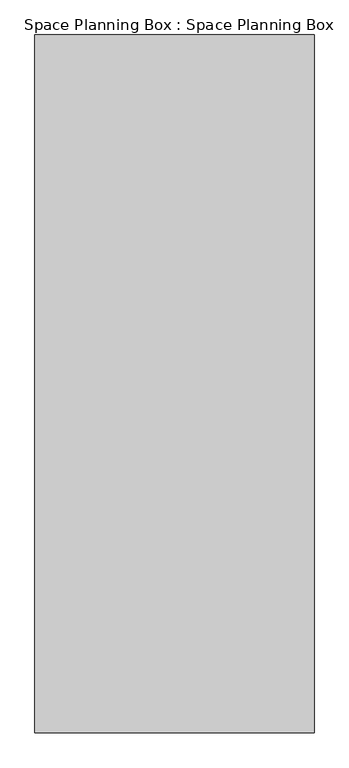
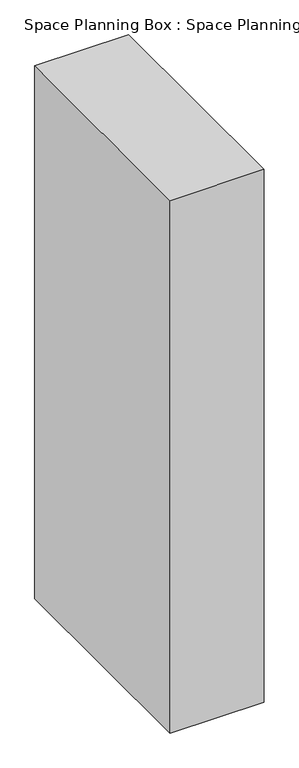
"""IFC4 building model written with IfcOpenShell, lengths in millimetres: proxy geometry, Space Planning Box : Space Planning Box."""

from ifc_helpers import new_model, si_unit, origin, origin_with_axes, place, context, project, spatial, polyline, outline, extrude, source, transform, mapped, element, save


def space_planning_box_space_planning_box_71e2440f(model_context):
    return source(origin(), model_context, "Body", "SweptSolid", [
        extrude(outline(polyline([(500.0, 1250.0), (500.0, -1250.0), (-500.0, -1250.0), (-500.0, 1250.0), (500.0, 1250.0)])), origin_with_axes(), (0.0, 0.0, 1.0), 6000.0),
    ])


if __name__ == "__main__":
    model = new_model("IFC4")
    model_context = context("Model", 3, world=origin())
    ifc_project = project(units=[si_unit("LENGTHUNIT", "METRE", prefix="MILLI")], contexts=[model_context])
    site = spatial("IfcSite", under=ifc_project)
    building = spatial("IfcBuilding", under=site)
    placement = place(None, origin())
    space_planning_box_space_planning_box_shape = space_planning_box_space_planning_box_71e2440f(model_context)
    element("IfcBuildingElementProxy", 1, Name="Space Planning Box : Space Planning Box", ObjectType="Space Planning Box : Space Planning Box", at=placement, inside=building, context=model_context, shape_type="MappedRepresentation", body=[
        mapped(space_planning_box_space_planning_box_shape, transform((0.0, 0.0, 0.0), x_axis=(1.0, 0.0, 0.0), y_axis=(0.0, 1.0, 0.0), z_axis=(0.0, 0.0, 1.0))),
    ])
    save(model, "model.ifc")

# Revit data of these elements
# Type "Space Planning Box : Space Planning Box"
#   Type Comments = "..."
#   Room Name [instance default] = "?"
#   Assembly Code = "..."
#   Width [instance default] = 1524 mm
#   Program Area [instance default] = 0 m²
#   Length [instance default] = 1524 mm
#   Height [instance default] = 1524 mm
#   Area [instance default] = 2.32258 m²
#   Fill Color [instance default] = Cyan
#   Default Elevation = 0
# Element 1 (IfcBuildingElementProxy, "Space Planning Box : Space Planning Box")
#   Room Name = "Pipe Shaft"
#   Width = 1000 mm
#   Program Area = 2.5 m²
#   Length = 2500 mm
#   Height = 6000 mm
#   Area = 2.5 m²
#   Fill Color = Pink
#   Materials on its faces: "Pink"
# Materials
#   "Cyan": class "Generic", colour RGB 0 255 255, transparency 0.2, Cost = 0
#   "Pink": class "Generic", colour RGB 255 105 180, transparency 0.2, Cost = 0
